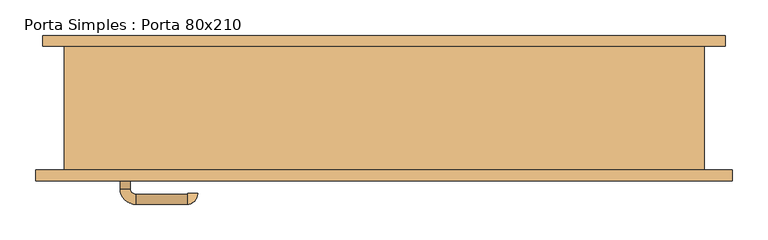
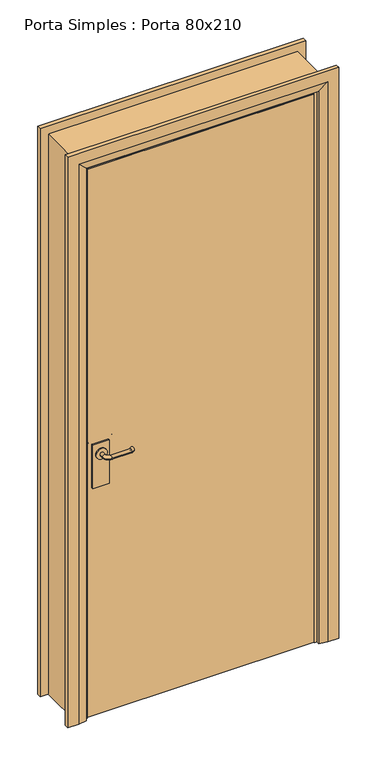
"""IFC4 building model written with IfcOpenShell, lengths in millimetres: door geometry, Porta Simples : Porta 80x210."""

import ifcopenshell
import ifcopenshell.guid

model = None  # the IFC model being written
_history = None  # IfcOwnerHistory: only IFC2X3 demands one
_inside = {}  # id of a spatial element -> (the spatial element, [elements in it])
_under = {}  # id of a project, library or spatial element -> (it, [spatial elements below it])
_declared = {}  # id of a project -> (the project, [libraries it declares])
_typed = {}  # id of a type object -> (the type object, [elements of that type])
_made_of = {}  # id of a material, layer set ... -> (it, [elements and type objects made of it])


def new_model(schema):
    """Start an empty IFC model of exactly this schema.

    Asked for "IFC4X3", IfcOpenShell would pick the latest addendum, in which some entities
    have other attributes; the version numbers below select the first issue.
    IFC2X3 requires an IfcOwnerHistory on every rooted entity: one is made here for all.
    """
    global model, _history
    if schema == "IFC4X3":
        model = ifcopenshell.file(schema_version=(4, 3, 0, 0))
    else:
        model = ifcopenshell.file(schema=schema)
    _inside.clear()
    _under.clear()
    _declared.clear()
    _typed.clear()
    _made_of.clear()
    _history = None
    if model.schema == "IFC2X3":
        org = make("IfcOrganization", Name="unknown")
        user = make(
            "IfcPersonAndOrganization",
            ThePerson=make("IfcPerson", FamilyName="unknown"),
            TheOrganization=org,
        )
        app = make(
            "IfcApplication",
            ApplicationDeveloper=org,
            Version="unknown",
            ApplicationFullName="unknown",
            ApplicationIdentifier="unknown",
        )
        _history = make(
            "IfcOwnerHistory",
            OwningUser=user,
            OwningApplication=app,
            ChangeAction="ADDED",
            CreationDate=0,
        )
    return model


def make(cls, **values):
    """One entity of the class cls with the attributes given. An attribute that is None is left unset."""
    return model.create_entity(
        cls, **{name: value for name, value in values.items() if value is not None}
    )


def rooted(cls, **values):
    """An entity with a GlobalId (a new one), such as an element, a storey or a relation."""
    return make(cls, GlobalId=ifcopenshell.guid.new(), OwnerHistory=_history, **values)


def si_unit(unit_type, name, prefix=None):
    """IfcSIUnit, for example si_unit("LENGTHUNIT", "METRE", prefix="MILLI")."""
    return make("IfcSIUnit", UnitType=unit_type, Prefix=prefix, Name=name)


def assignment(units):
    """IfcUnitAssignment: the units of a project."""
    return None if units is None else make("IfcUnitAssignment", Units=units)


def point(xyz):
    """IfcCartesianPoint."""
    return None if xyz is None else make("IfcCartesianPoint", Coordinates=xyz)


def direction(xyz):
    """IfcDirection."""
    return None if xyz is None else make("IfcDirection", DirectionRatios=xyz)


def frame(location, z_axis=None, x_axis=None):
    """IfcAxis2Placement3D, a coordinate frame: its origin and axes. An axis left out is left unset."""
    return make(
        "IfcAxis2Placement3D",
        Location=point(location),
        Axis=direction(z_axis),
        RefDirection=direction(x_axis),
    )


def frame_2d(location, x_axis=None):
    """IfcAxis2Placement2D, a coordinate frame in the plane: its origin and x axis."""
    return make(
        "IfcAxis2Placement2D", Location=point(location), RefDirection=direction(x_axis)
    )


def origin():
    """The frame at (0, 0, 0) with its axes left unset."""
    return frame((0.0, 0.0, 0.0))


def place(relative_to, where):
    """IfcLocalPlacement: puts the frame where relative to a parent placement (None: the world)."""
    return make(
        "IfcLocalPlacement", PlacementRelTo=relative_to, RelativePlacement=where
    )


def context(
    kind, dimensions, precision=None, world=None, true_north=None, identifier=None
):
    """IfcGeometricRepresentationContext, for example the 3D "Model" context."""
    return make(
        "IfcGeometricRepresentationContext",
        ContextIdentifier=identifier,
        ContextType=kind,
        CoordinateSpaceDimension=dimensions,
        Precision=precision,
        WorldCoordinateSystem=world,
        TrueNorth=true_north,
    )


def project(units=None, contexts=None):
    """IfcProject with its units and contexts."""
    return rooted(
        "IfcProject",
        Name="project",
        RepresentationContexts=contexts,
        UnitsInContext=assignment(units),
    )


def spatial(cls, under=None, at=None, **own):
    """A site, building, storey or space (cls), placed at a placement, below another one or the project."""
    s = rooted(cls, ObjectPlacement=at, **own)
    if under is not None:
        _under.setdefault(under.id(), (under, []))[1].append(s)
    return s


def polyline(points):
    """IfcPolyline through the points."""
    return make("IfcPolyline", Points=[point(p) for p in points])


def circle_curve(where, radius):
    """IfcCircle in the frame where."""
    return make("IfcCircle", Position=where, Radius=radius)


def ellipse_curve(where, semi_axis1, semi_axis2):
    """IfcEllipse in the frame where."""
    return make(
        "IfcEllipse", Position=where, SemiAxis1=semi_axis1, SemiAxis2=semi_axis2
    )


def trimmed(basis, trim1, trim2, sense, master):
    """IfcTrimmedCurve: the piece of a basis curve between two trims."""
    return make(
        "IfcTrimmedCurve",
        BasisCurve=basis,
        Trim1=trim1,
        Trim2=trim2,
        SenseAgreement=sense,
        MasterRepresentation=master,
    )


def segment(curve, same_sense, transition):
    """IfcCompositeCurveSegment."""
    return make(
        "IfcCompositeCurveSegment",
        Transition=transition,
        SameSense=same_sense,
        ParentCurve=curve,
    )


def composite_curve(segments, self_intersect=None):
    """IfcCompositeCurve: segments joined end to end."""
    return make("IfcCompositeCurve", Segments=segments, SelfIntersect=self_intersect)


def outline(outer, holes=None, kind="AREA"):
    """IfcArbitraryClosedProfileDef: a profile drawn as a closed curve; with holes, ...WithVoids."""
    if holes is None:
        return make("IfcArbitraryClosedProfileDef", ProfileType=kind, OuterCurve=outer)
    return make(
        "IfcArbitraryProfileDefWithVoids",
        ProfileType=kind,
        OuterCurve=outer,
        InnerCurves=holes,
    )


def extrude(swept, where, along, depth):
    """IfcExtrudedAreaSolid: the profile swept, set in the frame where, extruded along a direction by depth."""
    return make(
        "IfcExtrudedAreaSolid",
        SweptArea=swept,
        Position=where,
        ExtrudedDirection=direction(along),
        Depth=depth,
    )


def faces_of(points, faces, orient=None, outer=None):
    """IfcFace entities. A face is a list of loops; a loop is a list of indices into points, from 0.

    orient and outer hold one flag for each loop. By default every Orientation is true, the
    first loop of a face is its IfcFaceOuterBound and the others are IfcFaceBound.
    """
    made = []
    for i, loops in enumerate(faces):
        bounds = []
        for j, loop in enumerate(loops):
            is_outer = j == 0 if outer is None else outer[i][j]
            bounds.append(
                make(
                    "IfcFaceOuterBound" if is_outer else "IfcFaceBound",
                    Bound=make("IfcPolyLoop", Polygon=[points[k] for k in loop]),
                    Orientation=True if orient is None else orient[i][j],
                )
            )
        made.append(make("IfcFace", Bounds=bounds))
    return made


def faceted_brep(points, faces, orient=None, outer=None, voids=None):
    """IfcFacetedBrep: a solid bounded by flat faces; with voids (closed shells), ...WithVoids."""
    shared = [point(p) for p in points]
    hull = make("IfcClosedShell", CfsFaces=faces_of(shared, faces, orient, outer))
    if voids is None:
        return make("IfcFacetedBrep", Outer=hull)
    return make(
        "IfcFacetedBrepWithVoids",
        Outer=hull,
        Voids=[
            make(cls, CfsFaces=faces_of(shared, fs, o, b)) for cls, fs, o, b in voids
        ],
    )


def shape(context_of_items, identifier, shape_type, items):
    """IfcShapeRepresentation: the items that make up one representation, for example the "Body"."""
    return make(
        "IfcShapeRepresentation",
        ContextOfItems=context_of_items,
        RepresentationIdentifier=identifier,
        RepresentationType=shape_type,
        Items=items,
    )


def source(mapping_origin, context_of_items, identifier, shape_type, items):
    """IfcRepresentationMap: a shape defined once, which mapped items show again and again."""
    return make(
        "IfcRepresentationMap",
        MappingOrigin=mapping_origin,
        MappedRepresentation=shape(context_of_items, identifier, shape_type, items),
    )


def transform(
    local_origin,
    x_axis=None,
    y_axis=None,
    z_axis=None,
    scale=None,
    scale2=None,
    scale3=None,
    uniform=True,
):
    """IfcCartesianTransformationOperator3D, or its non-uniform kind. x_axis, y_axis, z_axis: its Axis1, 2, 3."""
    if uniform:
        return make(
            "IfcCartesianTransformationOperator3D",
            Axis1=direction(x_axis),
            Axis2=direction(y_axis),
            LocalOrigin=point(local_origin),
            Scale=scale,
            Axis3=direction(z_axis),
        )
    return make(
        "IfcCartesianTransformationOperator3DnonUniform",
        Axis1=direction(x_axis),
        Axis2=direction(y_axis),
        LocalOrigin=point(local_origin),
        Scale=scale,
        Axis3=direction(z_axis),
        Scale2=scale2,
        Scale3=scale3,
    )


def mapped(mapping_source, mapping_target):
    """IfcMappedItem: shows the shape of a source again, moved by a transform."""
    return make(
        "IfcMappedItem", MappingSource=mapping_source, MappingTarget=mapping_target
    )


def made_of(thing, what):
    """Note that an element or type object is made of a material, layer set ...; save() writes the relation."""
    if what is not None:
        _made_of.setdefault(what.id(), (what, []))[1].append(thing)
    return thing


def element(
    cls,
    number,
    at=None,
    inside=None,
    cuts=None,
    type_object=None,
    material=None,
    context=None,
    identifier="Body",
    shape_type=None,
    held_by="IfcProductDefinitionShape",
    body=None,
    shapes=None,
    **own,
):
    """One element of the class cls, such as IfcWall. Its Tag is "e" and its number.

    at: its placement. inside: the storey or other place that contains it. cuts: it is an
    opening in that element (IfcRelVoidsElement). A single representation is given by context,
    identifier, shape_type and body (its items); several are given by shapes. held_by: the class
    of the entity that holds the representations. save() writes the other relations.
    """
    e = rooted(cls, Tag="e%d" % number, ObjectPlacement=at, **own)
    if body is not None:
        shapes = [shape(context, identifier, shape_type, body)]
    if shapes is not None:
        e.Representation = make(held_by, Representations=shapes)
    if inside is not None:
        _inside.setdefault(inside.id(), (inside, []))[1].append(e)
    if cuts is not None:
        rooted(
            "IfcRelVoidsElement", RelatingBuildingElement=cuts, RelatedOpeningElement=e
        )
    if type_object is not None:
        _typed.setdefault(type_object.id(), (type_object, []))[1].append(e)
    return made_of(e, material)


def aggregate(whole, parts):
    """IfcRelAggregates: a whole, such as a stair, and the parts it consists of."""
    return rooted("IfcRelAggregates", RelatingObject=whole, RelatedObjects=parts)


def save(model, path):
    """Write the relations noted so far, then the file.

    IfcRelAggregates (storeys below a building ...), IfcRelContainedInSpatialStructure (elements
    in a storey), IfcRelDefinesByType, IfcRelAssociatesMaterial and IfcRelDeclares: one each for
    every whole, place, type object, material and project.
    """
    for whole, parts in _under.values():
        aggregate(whole, parts)
    for where, things in _inside.values():
        rooted(
            "IfcRelContainedInSpatialStructure",
            RelatedElements=things,
            RelatingStructure=where,
        )
    for kind, things in _typed.values():
        rooted("IfcRelDefinesByType", RelatedObjects=things, RelatingType=kind)
    for what, things in _made_of.values():
        rooted("IfcRelAssociatesMaterial", RelatedObjects=things, RelatingMaterial=what)
    for by, libraries in _declared.values():
        rooted("IfcRelDeclares", RelatingContext=by, RelatedDefinitions=libraries)
    model.write(path)


def plane_surface(at):
    """IfcPlane: the flat surface through the origin of the frame at, square to its z axis."""
    return make("IfcPlane", Position=at)


def cylinder_surface(at, radius):
    """IfcCylindricalSurface: all points at the distance radius from the z axis of the frame at."""
    return make("IfcCylindricalSurface", Position=at, Radius=radius)


def revolved_surface(curve, axis_point, axis_direction):
    """IfcSurfaceOfRevolution: the curve turned about the line through axis_point along axis_direction."""
    return make(
        "IfcSurfaceOfRevolution",
        SweptCurve=make("IfcArbitraryOpenProfileDef", ProfileType="CURVE", Curve=curve),
        AxisPosition=make("IfcAxis1Placement", Location=point(axis_point), Axis=direction(axis_direction)),
    )


def advanced_brep(points, edges, surfaces, faces):
    """IfcAdvancedBrep: a solid bounded by faces that lie on surfaces and meet in shared edges.

    An edge is (start, end): straight between two places in points (the first is 0);
    or (start, end, curve); or (start, end, curve, False) where it runs against its curve.
    A face is (place in surfaces, loops), or (place, loops, False) where it looks against
    its surface's normal. A loop lists edges by number (the first is 1), with a minus sign
    where the edge is run from its end to its start. The first loop is the outer one.
    """
    corners = [point(p) for p in points]
    vertices = [make("IfcVertexPoint", VertexGeometry=c) for c in corners]
    made = []
    for start, end, *more in edges:
        made.append(
            make(
                "IfcEdgeCurve",
                EdgeStart=vertices[start],
                EdgeEnd=vertices[end],
                EdgeGeometry=more[0] if more else make("IfcPolyline", Points=[corners[start], corners[end]]),
                SameSense=more[1] if len(more) > 1 else True,
            )
        )
    hull = []
    for where, loops, *sense in faces:
        bounds = []
        for j, loop in enumerate(loops):
            ring = [make("IfcOrientedEdge", EdgeElement=made[abs(k) - 1], Orientation=k > 0) for k in loop]
            bounds.append(
                make(
                    "IfcFaceOuterBound" if j == 0 else "IfcFaceBound",
                    Bound=make("IfcEdgeLoop", EdgeList=ring),
                    Orientation=True,
                )
            )
        hull.append(make("IfcAdvancedFace", Bounds=bounds, FaceSurface=surfaces[where], SameSense=sense[0] if sense else True))
    return make("IfcAdvancedBrep", Outer=make("IfcClosedShell", CfsFaces=hull))


def porta_simples_porta_80x210_20d964b4(model_context):
    return source(origin(), model_context, "Body", "SolidModel", [
        extrude(outline(composite_curve([segment(trimmed(circle_curve(frame_2d((1050.0, -364.0)), 20.0), [point((1050.0, -384.0))], [point((1050.0, -344.0))], False, "CARTESIAN"), True, "CONTINUOUS"), segment(trimmed(circle_curve(frame_2d((1050.0, -364.0)), 20.0), [point((1050.0, -344.0))], [point((1050.0, -384.0))], False, "CARTESIAN"), True, "CONTINUOUS")], self_intersect=False)), frame((0.0, -46.3, 0.0), z_axis=(0.0, 1.0, 0.0), x_axis=(0.0, 0.0, 1.0)), (0.0, 0.0, 1.0), 4.5929895),
        advanced_brep(
        [(-357.0, -41.7070105, 1050.0), (-371.0, -41.7070105, 1050.0), (-357.0, -26.3, 1050.0), (-371.0, -26.3, 1050.0), (-349.0, -4.3, 1050.0), (-349.0, -18.3, 1050.0), (-277.0, -18.3, 1050.0), (-277.0, -4.3, 1050.0), (-276.0, -19.3, 1050.0), (-262.0, -19.3, 1050.0)],
        [
            (0, 1, circle_curve(frame((-364.0, -41.7070105, 1050.0), z_axis=(0.0, -1.0, 0.0), x_axis=(-1.0, 0.0, 0.0)), 7.0)),
            (1, 0, circle_curve(frame((-364.0, -41.7070105, 1050.0), z_axis=(0.0, -1.0, 0.0), x_axis=(-1.0, 0.0, 0.0)), 7.0)),
            (0, 2),
            (2, 3, circle_curve(frame((-364.0, -26.3, 1050.0), z_axis=(0.0, -1.0, 0.0), x_axis=(-1.0, 0.0, 0.0)), 7.0)),
            (3, 1),
            (3, 2, circle_curve(frame((-364.0, -26.3, 1050.0), z_axis=(0.0, -1.0, 0.0), x_axis=(-1.0, 0.0, 0.0)), 7.0)),
            (4, 3, circle_curve(frame((-349.0, -26.3, 1050.0), z_axis=(0.0, 0.0, 1.0), x_axis=(-1.0, 0.0, 0.0)), 22.0)),
            (2, 5, circle_curve(frame((-349.0, -26.3, 1050.0), z_axis=(0.0, 0.0, -1.0), x_axis=(-1.0, 0.0, 0.0)), 8.0)),
            (5, 4, circle_curve(frame((-349.0, -11.3, 1050.0), z_axis=(-1.0, 0.0, 0.0), x_axis=(0.0, 1.0, 0.0)), 7.0)),
            (4, 5, circle_curve(frame((-349.0, -11.3, 1050.0), z_axis=(-1.0, 0.0, 0.0), x_axis=(0.0, 1.0, 0.0)), 7.0)),
            (5, 6),
            (6, 7, circle_curve(frame((-277.0, -11.3, 1050.0), z_axis=(-1.0, 0.0, 0.0), x_axis=(0.0, 1.0, 0.0)), 7.0)),
            (7, 4),
            (7, 6, circle_curve(frame((-277.0, -11.3, 1050.0), z_axis=(-1.0, 0.0, 0.0), x_axis=(0.0, 1.0, 0.0)), 7.0)),
            (8, 9, circle_curve(frame((-269.0, -19.3, 1050.0), z_axis=(0.0, -1.0, 0.0), x_axis=(1.0, 0.0, 0.0)), 7.0)),
            (9, 8, circle_curve(frame((-269.0, -19.3, 1050.0), z_axis=(0.0, -1.0, 0.0), x_axis=(1.0, 0.0, 0.0)), 7.0)),
            (9, 7, circle_curve(frame((-277.0, -19.3, 1050.0), z_axis=(0.0, 0.0, 1.0), x_axis=(0.0, 1.0, 0.0)), 15.0)),
            (6, 8, circle_curve(frame((-277.0, -19.3, 1050.0), z_axis=(0.0, 0.0, -1.0), x_axis=(0.0, 1.0, 0.0)), 1.0)),
        ],
        [
            plane_surface(frame((-364.0, -41.7070105, 1050.0), z_axis=(0.0, -1.0, 0.0), x_axis=(0.0, 0.0, 1.0))),
            cylinder_surface(frame((-364.0, -41.7070105, 1050.0), z_axis=(0.0, -1.0, 0.0), x_axis=(-1.0, 0.0, 0.0)), 7.0),
            revolved_surface(trimmed(ellipse_curve(frame((-364.0, -26.3, 1050.0), z_axis=(0.0, -1.0, 0.0), x_axis=(-1.0, 0.0, 0.0)), 7.0, 7.0), [point((-357.0, -26.3, 1050.0))], [point((-371.0, -26.3, 1050.0))], True, "CARTESIAN"), (-349.0, -26.3, 1050.0), (0.0, 0.0, -1.0)),
            revolved_surface(trimmed(ellipse_curve(frame((-364.0, -26.3, 1050.0), z_axis=(0.0, -1.0, 0.0), x_axis=(-1.0, 0.0, 0.0)), 7.0, 7.0), [point((-371.0, -26.3, 1050.0))], [point((-357.0, -26.3, 1050.0))], True, "CARTESIAN"), (-349.0, -26.3, 1050.0), (0.0, 0.0, -1.0)),
            cylinder_surface(frame((-349.0, -11.3, 1050.0), z_axis=(-1.0, 0.0, 0.0), x_axis=(0.0, 1.0, 0.0)), 7.0),
            plane_surface(frame((-269.0, -19.3, 1050.0), z_axis=(0.0, -1.0, 0.0), x_axis=(0.0, 0.0, 1.0))),
            revolved_surface(trimmed(ellipse_curve(frame((-277.0, -11.3, 1050.0), z_axis=(-1.0, 0.0, 0.0), x_axis=(0.0, 1.0, 0.0)), 7.0, 7.0), [point((-277.0, -18.3, 1050.0))], [point((-277.0, -4.3, 1050.0))], True, "CARTESIAN"), (-277.0, -19.3, 1050.0), (0.0, 0.0, -1.0)),
            revolved_surface(trimmed(ellipse_curve(frame((-277.0, -11.3, 1050.0), z_axis=(-1.0, 0.0, 0.0), x_axis=(0.0, 1.0, 0.0)), 7.0, 7.0), [point((-277.0, -4.3, 1050.0))], [point((-277.0, -18.3, 1050.0))], True, "CARTESIAN"), (-277.0, -19.3, 1050.0), (0.0, 0.0, -1.0)),
        ],
        [
            (0, [[1, 2]]),
            (1, [[-1, 3, 4, 5]]),
            (1, [[-2, -5, 6, -3]]),
            (2, [[7, -4, 8, 9]]),
            (3, [[-8, -6, -7, 10]]),
            (4, [[-9, 11, 12, 13]]),
            (4, [[-10, -13, 14, -11]]),
            (5, [[15, 16]]),
            (6, [[17, -12, 18, -16]]),
            (7, [[-18, -14, -17, -15]]),
        ],
    ),
        extrude(outline(polyline([(-334.0, -52.3), (-394.0, -52.3), (-394.0, -46.3), (-334.0, -46.3), (-334.0, -52.3)])), frame((0.0, 0.0, 925.0), z_axis=(0.0, 0.0, 1.0), x_axis=(1.0, 0.0, 0.0)), (0.0, 0.0, 1.0), 165.0),
        extrude(outline(composite_curve([segment(trimmed(circle_curve(frame_2d((1050.0, -364.0)), 20.0), [point((1050.0, -384.0))], [point((1050.0, -344.0))], False, "CARTESIAN"), True, "CONTINUOUS"), segment(trimmed(circle_curve(frame_2d((1050.0, -364.0)), 20.0), [point((1050.0, -344.0))], [point((1050.0, -384.0))], False, "CARTESIAN"), True, "CONTINUOUS")], self_intersect=False)), frame((0.0, -97.8929895, 0.0), z_axis=(0.0, 1.0, 0.0), x_axis=(0.0, 0.0, 1.0)), (0.0, 0.0, 1.0), 4.5929895),
        advanced_brep(
        [(-357.0, -97.8929895, 1050.0), (-371.0, -97.8929895, 1050.0), (-371.0, -113.3, 1050.0), (-357.0, -113.3, 1050.0), (-349.0, -135.3, 1050.0), (-349.0, -121.3, 1050.0), (-277.0, -135.3, 1050.0), (-277.0, -121.3, 1050.0), (-276.0, -120.3, 1050.0), (-262.0, -120.3, 1050.0)],
        [
            (0, 1, circle_curve(frame((-364.0, -97.8929895, 1050.0), z_axis=(0.0, 1.0, 0.0), x_axis=(-1.0, 0.0, 0.0)), 7.0)),
            (1, 0, circle_curve(frame((-364.0, -97.8929895, 1050.0), z_axis=(0.0, 1.0, 0.0), x_axis=(-1.0, 0.0, 0.0)), 7.0)),
            (1, 2),
            (2, 3, circle_curve(frame((-364.0, -113.3, 1050.0), z_axis=(0.0, 1.0, 0.0), x_axis=(-1.0, 0.0, 0.0)), 7.0)),
            (3, 0),
            (3, 2, circle_curve(frame((-364.0, -113.3, 1050.0), z_axis=(0.0, 1.0, 0.0), x_axis=(-1.0, 0.0, 0.0)), 7.0)),
            (4, 5, circle_curve(frame((-349.0, -128.3, 1050.0), z_axis=(-1.0, 0.0, 0.0), x_axis=(0.0, -1.0, 0.0)), 7.0)),
            (5, 3, circle_curve(frame((-349.0, -113.3, 1050.0), z_axis=(0.0, 0.0, -1.0), x_axis=(-1.0, 0.0, 0.0)), 8.0)),
            (2, 4, circle_curve(frame((-349.0, -113.3, 1050.0), z_axis=(0.0, 0.0, 1.0), x_axis=(-1.0, 0.0, 0.0)), 22.0)),
            (5, 4, circle_curve(frame((-349.0, -128.3, 1050.0), z_axis=(-1.0, 0.0, 0.0), x_axis=(0.0, -1.0, 0.0)), 7.0)),
            (4, 6),
            (6, 7, circle_curve(frame((-277.0, -128.3, 1050.0), z_axis=(-1.0, 0.0, 0.0), x_axis=(0.0, -1.0, 0.0)), 7.0)),
            (7, 5),
            (7, 6, circle_curve(frame((-277.0, -128.3, 1050.0), z_axis=(-1.0, 0.0, 0.0), x_axis=(0.0, -1.0, 0.0)), 7.0)),
            (8, 9, circle_curve(frame((-269.0, -120.3, 1050.0), z_axis=(0.0, 1.0, 0.0), x_axis=(1.0, 0.0, 0.0)), 7.0)),
            (9, 8, circle_curve(frame((-269.0, -120.3, 1050.0), z_axis=(0.0, 1.0, 0.0), x_axis=(1.0, 0.0, 0.0)), 7.0)),
            (8, 7, circle_curve(frame((-277.0, -120.3, 1050.0), z_axis=(0.0, 0.0, -1.0), x_axis=(0.0, -1.0, 0.0)), 1.0)),
            (6, 9, circle_curve(frame((-277.0, -120.3, 1050.0), z_axis=(0.0, 0.0, 1.0), x_axis=(0.0, -1.0, 0.0)), 15.0)),
        ],
        [
            plane_surface(frame((-364.0, -97.8929895, 1050.0), z_axis=(0.0, 1.0, 0.0), x_axis=(0.0, 0.0, 1.0))),
            cylinder_surface(frame((-364.0, -97.8929895, 1050.0), z_axis=(0.0, 1.0, 0.0), x_axis=(-1.0, 0.0, 0.0)), 7.0),
            revolved_surface(trimmed(ellipse_curve(frame((-364.0, -113.3, 1050.0), z_axis=(0.0, -1.0, 0.0), x_axis=(-1.0, 0.0, 0.0)), 7.0, 7.0), [point((-357.0, -113.3, 1050.0))], [point((-371.0, -113.3, 1050.0))], True, "CARTESIAN"), (-349.0, -113.3, 1050.0), (0.0, 0.0, -1.0)),
            revolved_surface(trimmed(ellipse_curve(frame((-364.0, -113.3, 1050.0), z_axis=(0.0, -1.0, 0.0), x_axis=(-1.0, 0.0, 0.0)), 7.0, 7.0), [point((-371.0, -113.3, 1050.0))], [point((-357.0, -113.3, 1050.0))], True, "CARTESIAN"), (-349.0, -113.3, 1050.0), (0.0, 0.0, -1.0)),
            cylinder_surface(frame((-349.0, -128.3, 1050.0), z_axis=(-1.0, 0.0, 0.0), x_axis=(0.0, -1.0, 0.0)), 7.0),
            plane_surface(frame((-269.0, -120.3, 1050.0), z_axis=(0.0, 1.0, 0.0), x_axis=(0.0, 0.0, 1.0))),
            revolved_surface(trimmed(ellipse_curve(frame((-277.0, -128.3, 1050.0), z_axis=(1.0, 0.0, 0.0), x_axis=(0.0, -1.0, 0.0)), 7.0, 7.0), [point((-277.0, -121.3, 1050.0))], [point((-277.0, -135.3, 1050.0))], True, "CARTESIAN"), (-277.0, -120.3, 1050.0), (0.0, 0.0, -1.0)),
            revolved_surface(trimmed(ellipse_curve(frame((-277.0, -128.3, 1050.0), z_axis=(1.0, 0.0, 0.0), x_axis=(0.0, -1.0, 0.0)), 7.0, 7.0), [point((-277.0, -135.3, 1050.0))], [point((-277.0, -121.3, 1050.0))], True, "CARTESIAN"), (-277.0, -120.3, 1050.0), (0.0, 0.0, -1.0)),
        ],
        [
            (0, [[1, 2]]),
            (1, [[3, 4, 5, -2]]),
            (1, [[-5, 6, -3, -1]]),
            (2, [[7, 8, -4, 9]]),
            (3, [[10, -9, -6, -8]]),
            (4, [[11, 12, 13, -7]]),
            (4, [[-13, 14, -11, -10]]),
            (5, [[15, 16]]),
            (6, [[-15, 17, -12, 18]]),
            (7, [[-16, -18, -14, -17]]),
        ],
    ),
        extrude(outline(polyline([(-334.0, -87.3), (-334.0, -93.3), (-394.0, -93.3), (-394.0, -87.3), (-334.0, -87.3)])), frame((0.0, 0.0, 925.0), z_axis=(0.0, 0.0, 1.0), x_axis=(1.0, 0.0, 0.0)), (0.0, 0.0, 1.0), 165.0),
        extrude(outline(polyline([(408.0, -52.3), (408.0, -87.3), (-408.0, -87.3), (-408.0, -52.3), (408.0, -52.3)])), frame((0.0, 0.0, 53.0), z_axis=(0.0, 0.0, 1.0), x_axis=(1.0, 0.0, 0.0)), (0.0, 0.0, 1.0), 2094.0),
        faceted_brep([(480.0, 87.3, 50.0), (410.0, 87.3, 50.0), (410.0, 97.3, 50.0), (440.0, 102.3, 50.0), (480.0, 102.3, 50.0), (480.0, 102.3, 2220.0), (480.0, 87.3, 2220.0), (440.0, 102.3, 2180.0), (-440.0, 102.3, 2180.0), (-440.0, 102.3, 50.0), (-480.0, 102.3, 50.0), (-480.0, 102.3, 2220.0), (410.0, 97.3, 2150.0), (410.0, 87.3, 2150.0), (-480.0, 87.3, 2220.0), (-480.0, 87.3, 50.0), (-410.0, 87.3, 50.0), (-410.0, 87.3, 2150.0), (-410.0, 97.3, 50.0), (-410.0, 97.3, 2150.0)], [[[0, 1, 2, 3, 4]], [[4, 5, 6, 0]], [[3, 7, 8, 9, 10, 11, 5, 4]], [[2, 12, 7, 3]], [[1, 13, 12, 2]], [[0, 6, 14, 15, 16, 17, 13, 1]], [[17, 16, 18, 19]], [[15, 10, 9, 18, 16]], [[11, 10, 15, 14]], [[19, 18, 9, 8]], [[13, 17, 19, 12]], [[5, 11, 14, 6]], [[12, 19, 8, 7]]]),
        faceted_brep([(490.0, -87.3, 50.0), (490.0, -102.3, 50.0), (450.0, -102.3, 50.0), (420.0, -97.3, 50.0), (420.0, -87.3, 50.0), (420.0, -87.3, 2160.0), (-420.0, -87.3, 2160.0), (-420.0, -87.3, 50.0), (-490.0, -87.3, 50.0), (-490.0, -87.3, 2230.0), (490.0, -87.3, 2230.0), (420.0, -97.3, 2160.0), (450.0, -102.3, 2190.0), (490.0, -102.3, 2230.0), (-490.0, -102.3, 2230.0), (-490.0, -102.3, 50.0), (-450.0, -102.3, 50.0), (-450.0, -102.3, 2190.0), (-420.0, -97.3, 50.0), (-420.0, -97.3, 2160.0)], [[[0, 1, 2, 3, 4]], [[4, 5, 6, 7, 8, 9, 10, 0]], [[3, 11, 5, 4]], [[2, 12, 11, 3]], [[1, 13, 14, 15, 16, 17, 12, 2]], [[0, 10, 13, 1]], [[9, 8, 15, 14]], [[8, 7, 18, 16, 15]], [[19, 18, 7, 6]], [[17, 16, 18, 19]], [[11, 19, 6, 5]], [[10, 9, 14, 13]], [[12, 17, 19, 11]]]),
        faceted_brep([(-410.0, -87.3, 50.0), (-450.0, -87.3, 50.0), (-450.0, 87.3, 50.0), (-400.0, 87.3, 50.0), (-400.0, -50.3, 50.0), (-410.0, -50.3, 50.0), (-410.0, -50.3, 2150.0), (-410.0, -87.3, 2150.0), (-400.0, -50.3, 2140.0), (-400.0, 87.3, 2140.0), (-450.0, 87.3, 2190.0), (-450.0, -87.3, 2190.0), (410.0, -87.3, 50.0), (410.0, -50.3, 50.0), (400.0, -50.3, 50.0), (400.0, 87.3, 50.0), (450.0, 87.3, 50.0), (450.0, -87.3, 50.0), (410.0, -87.3, 2150.0), (450.0, -87.3, 2190.0), (450.0, 87.3, 2190.0), (400.0, 87.3, 2140.0), (400.0, -50.3, 2140.0), (410.0, -50.3, 2150.0)], [[[0, 1, 2, 3, 4, 5]], [[5, 6, 7, 0]], [[4, 8, 6, 5]], [[3, 9, 8, 4]], [[2, 10, 9, 3]], [[1, 11, 10, 2]], [[0, 7, 11, 1]], [[12, 13, 14, 15, 16, 17]], [[18, 12, 17, 19]], [[19, 17, 16, 20]], [[20, 16, 15, 21]], [[21, 15, 14, 22]], [[22, 14, 13, 23]], [[23, 13, 12, 18]], [[6, 23, 18, 7]], [[8, 22, 23, 6]], [[9, 21, 22, 8]], [[10, 20, 21, 9]], [[11, 19, 20, 10]], [[7, 18, 19, 11]]]),
    ])


if __name__ == "__main__":
    model = new_model("IFC4")
    model_context = context("Model", 3, world=origin())
    ifc_project = project(units=[si_unit("LENGTHUNIT", "METRE", prefix="MILLI")], contexts=[model_context])
    site = spatial("IfcSite", under=ifc_project)
    building = spatial("IfcBuilding", under=site)
    placement = place(None, origin())
    porta_simples_porta_80x210_shape = porta_simples_porta_80x210_20d964b4(model_context)
    element("IfcDoor", 1, ObjectType="Porta Simples : Porta 80x210", at=placement, inside=building, context=model_context, shape_type="MappedRepresentation", body=[
        mapped(porta_simples_porta_80x210_shape, transform((0.0, 0.0, 0.0), x_axis=(1.0, 0.0, 0.0), y_axis=(0.0, 1.0, 0.0), z_axis=(0.0, 0.0, 1.0))),
    ])
    save(model, "model.ifc")

# Revit data of these elements
# Type "Porta Simples : Porta 80x210"
#   Type Mark = "49"
#   SINAPI = ""
#   Analytic Construction = "<Nenhum>"
#   Construction Type = "300"
#   Maçaneta [instance default] = ""
#   Fechadura [instance default] = ""
#   Vão Luz (somente para informação) = 0.78 m
#   Tolerância Folha Vertical = 0.003 m
#   Módulo Básico M = 0.10 m
#   Largura de Coordenação Modular Largura CM = 0.90 m
#   Rough Width = 0.90 m
#   Deslocamento da Horizontal da Folha = 0.00 m
#   Altura de Coordenação Modular Largura CM = 2.20 m
#   Rough Height = 2.20 m
#   Altura Nominal = 2.09 m
#   Ajuste de Coordenação Topo AC Topo = 0.01 m
#   Ajuste de Coordenação Base AC Base = 0.05 m
#   Ajuste de Coordenação AC = 0.01 m
#   Tolerância Folha Horizontal = 0.002 m
#   Largura Folha (somente para informação) = 0.796 m
#   Espessura Folha = 0.035 m
#   Maçaneta - Distância da Folha = 0.044 m
#   Maçaneta - Altura = 1.00 m
#   Largura Nominal (Largura Mn) = 0.82 m
#   Distância do Nível = 0.003 m
#   Aduela Interna Espessura = 0.04 m
#   Aduela Externa Espessura = 0.05 m
#   Altura Folha (somente para informação) = 2.075 m
#   Height = 2.14 m
#   Width = 0.88 m
#   Número de Módulos Básicos nM Largura = 9
#   Número de Módulos Básicos nM Altura = 22
#   Marco Metálico = no
#   Aduela de Madeira = no
#   Aduela Metálica de Canto = no
#   Guarnição Reta = no
#   Guarnição Chanfrada = yes
#   Batente - Material [instance default] = none
#   Painel - Material [instance default] = none
#   Model = ""
#   Function = (empty or 0)
#   Description = (empty or 0)
#   Wall Closure = (empty or 0)
#   Assembly Code = ""
# Element 1 (IfcDoor, "Porta Simples : Porta 80x210")
#   Materials on its faces: "Porta - Maçaneta"
# Materials
#   "Porta - Maçaneta": class "Diversos", colour RGB 0 0 0, transparency 0
